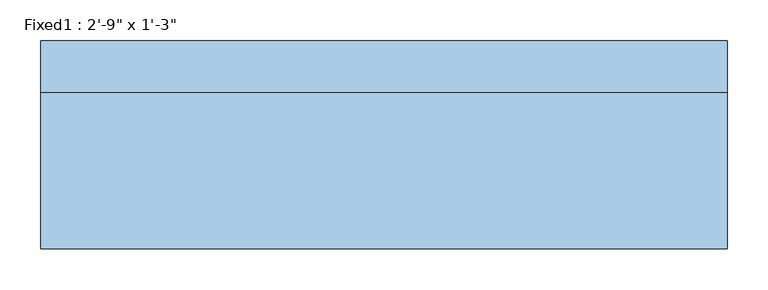
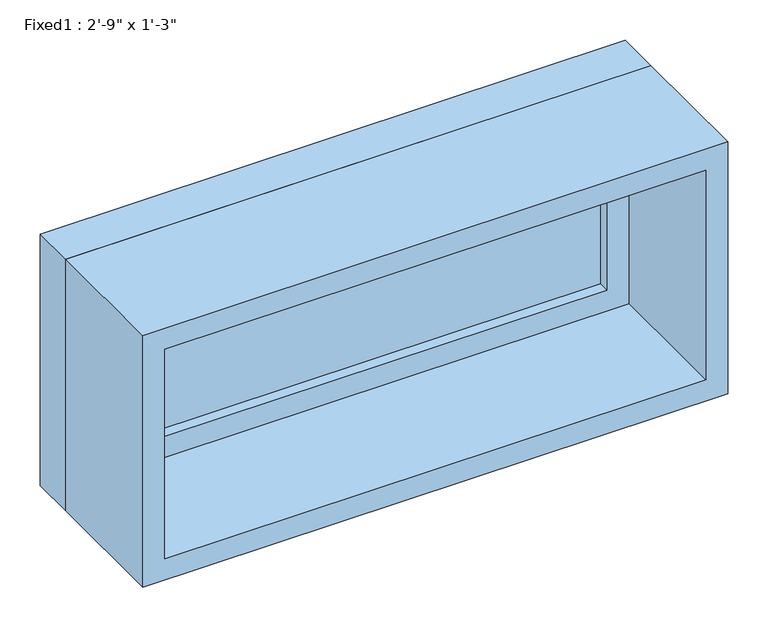
"""IFC4 building model written with IfcOpenShell, lengths in millimetres: window geometry."""

import ifcopenshell
import ifcopenshell.guid

model = None  # the IFC model being written
_history = None  # IfcOwnerHistory: only IFC2X3 demands one
_inside = {}  # id of a spatial element -> (the spatial element, [elements in it])
_under = {}  # id of a project, library or spatial element -> (it, [spatial elements below it])
_declared = {}  # id of a project -> (the project, [libraries it declares])
_typed = {}  # id of a type object -> (the type object, [elements of that type])
_made_of = {}  # id of a material, layer set ... -> (it, [elements and type objects made of it])


def new_model(schema):
    """Start an empty IFC model of exactly this schema.

    Asked for "IFC4X3", IfcOpenShell would pick the latest addendum, in which some entities
    have other attributes; the version numbers below select the first issue.
    IFC2X3 requires an IfcOwnerHistory on every rooted entity: one is made here for all.
    """
    global model, _history
    if schema == "IFC4X3":
        model = ifcopenshell.file(schema_version=(4, 3, 0, 0))
    else:
        model = ifcopenshell.file(schema=schema)
    _inside.clear()
    _under.clear()
    _declared.clear()
    _typed.clear()
    _made_of.clear()
    _history = None
    if model.schema == "IFC2X3":
        org = make("IfcOrganization", Name="unknown")
        user = make(
            "IfcPersonAndOrganization",
            ThePerson=make("IfcPerson", FamilyName="unknown"),
            TheOrganization=org,
        )
        app = make(
            "IfcApplication",
            ApplicationDeveloper=org,
            Version="unknown",
            ApplicationFullName="unknown",
            ApplicationIdentifier="unknown",
        )
        _history = make(
            "IfcOwnerHistory",
            OwningUser=user,
            OwningApplication=app,
            ChangeAction="ADDED",
            CreationDate=0,
        )
    return model


def make(cls, **values):
    """One entity of the class cls with the attributes given. An attribute that is None is left unset."""
    return model.create_entity(
        cls, **{name: value for name, value in values.items() if value is not None}
    )


def rooted(cls, **values):
    """An entity with a GlobalId (a new one), such as an element, a storey or a relation."""
    return make(cls, GlobalId=ifcopenshell.guid.new(), OwnerHistory=_history, **values)


def si_unit(unit_type, name, prefix=None):
    """IfcSIUnit, for example si_unit("LENGTHUNIT", "METRE", prefix="MILLI")."""
    return make("IfcSIUnit", UnitType=unit_type, Prefix=prefix, Name=name)


def assignment(units):
    """IfcUnitAssignment: the units of a project."""
    return None if units is None else make("IfcUnitAssignment", Units=units)


def point(xyz):
    """IfcCartesianPoint."""
    return None if xyz is None else make("IfcCartesianPoint", Coordinates=xyz)


def direction(xyz):
    """IfcDirection."""
    return None if xyz is None else make("IfcDirection", DirectionRatios=xyz)


def frame(location, z_axis=None, x_axis=None):
    """IfcAxis2Placement3D, a coordinate frame: its origin and axes. An axis left out is left unset."""
    return make(
        "IfcAxis2Placement3D",
        Location=point(location),
        Axis=direction(z_axis),
        RefDirection=direction(x_axis),
    )


def origin():
    """The frame at (0, 0, 0) with its axes left unset."""
    return frame((0.0, 0.0, 0.0))


def place(relative_to, where):
    """IfcLocalPlacement: puts the frame where relative to a parent placement (None: the world)."""
    return make(
        "IfcLocalPlacement", PlacementRelTo=relative_to, RelativePlacement=where
    )


def context(
    kind, dimensions, precision=None, world=None, true_north=None, identifier=None
):
    """IfcGeometricRepresentationContext, for example the 3D "Model" context."""
    return make(
        "IfcGeometricRepresentationContext",
        ContextIdentifier=identifier,
        ContextType=kind,
        CoordinateSpaceDimension=dimensions,
        Precision=precision,
        WorldCoordinateSystem=world,
        TrueNorth=true_north,
    )


def project(units=None, contexts=None):
    """IfcProject with its units and contexts."""
    return rooted(
        "IfcProject",
        Name="project",
        RepresentationContexts=contexts,
        UnitsInContext=assignment(units),
    )


def spatial(cls, under=None, at=None, **own):
    """A site, building, storey or space (cls), placed at a placement, below another one or the project."""
    s = rooted(cls, ObjectPlacement=at, **own)
    if under is not None:
        _under.setdefault(under.id(), (under, []))[1].append(s)
    return s


def polyline(points):
    """IfcPolyline through the points."""
    return make("IfcPolyline", Points=[point(p) for p in points])


def outline(outer, holes=None, kind="AREA"):
    """IfcArbitraryClosedProfileDef: a profile drawn as a closed curve; with holes, ...WithVoids."""
    if holes is None:
        return make("IfcArbitraryClosedProfileDef", ProfileType=kind, OuterCurve=outer)
    return make(
        "IfcArbitraryProfileDefWithVoids",
        ProfileType=kind,
        OuterCurve=outer,
        InnerCurves=holes,
    )


def extrude(swept, where, along, depth):
    """IfcExtrudedAreaSolid: the profile swept, set in the frame where, extruded along a direction by depth."""
    return make(
        "IfcExtrudedAreaSolid",
        SweptArea=swept,
        Position=where,
        ExtrudedDirection=direction(along),
        Depth=depth,
    )


def shape(context_of_items, identifier, shape_type, items):
    """IfcShapeRepresentation: the items that make up one representation, for example the "Body"."""
    return make(
        "IfcShapeRepresentation",
        ContextOfItems=context_of_items,
        RepresentationIdentifier=identifier,
        RepresentationType=shape_type,
        Items=items,
    )


def source(mapping_origin, context_of_items, identifier, shape_type, items):
    """IfcRepresentationMap: a shape defined once, which mapped items show again and again."""
    return make(
        "IfcRepresentationMap",
        MappingOrigin=mapping_origin,
        MappedRepresentation=shape(context_of_items, identifier, shape_type, items),
    )


def transform(
    local_origin,
    x_axis=None,
    y_axis=None,
    z_axis=None,
    scale=None,
    scale2=None,
    scale3=None,
    uniform=True,
):
    """IfcCartesianTransformationOperator3D, or its non-uniform kind. x_axis, y_axis, z_axis: its Axis1, 2, 3."""
    if uniform:
        return make(
            "IfcCartesianTransformationOperator3D",
            Axis1=direction(x_axis),
            Axis2=direction(y_axis),
            LocalOrigin=point(local_origin),
            Scale=scale,
            Axis3=direction(z_axis),
        )
    return make(
        "IfcCartesianTransformationOperator3DnonUniform",
        Axis1=direction(x_axis),
        Axis2=direction(y_axis),
        LocalOrigin=point(local_origin),
        Scale=scale,
        Axis3=direction(z_axis),
        Scale2=scale2,
        Scale3=scale3,
    )


def mapped(mapping_source, mapping_target):
    """IfcMappedItem: shows the shape of a source again, moved by a transform."""
    return make(
        "IfcMappedItem", MappingSource=mapping_source, MappingTarget=mapping_target
    )


def made_of(thing, what):
    """Note that an element or type object is made of a material, layer set ...; save() writes the relation."""
    if what is not None:
        _made_of.setdefault(what.id(), (what, []))[1].append(thing)
    return thing


def element(
    cls,
    number,
    at=None,
    inside=None,
    cuts=None,
    type_object=None,
    material=None,
    context=None,
    identifier="Body",
    shape_type=None,
    held_by="IfcProductDefinitionShape",
    body=None,
    shapes=None,
    **own,
):
    """One element of the class cls, such as IfcWall. Its Tag is "e" and its number.

    at: its placement. inside: the storey or other place that contains it. cuts: it is an
    opening in that element (IfcRelVoidsElement). A single representation is given by context,
    identifier, shape_type and body (its items); several are given by shapes. held_by: the class
    of the entity that holds the representations. save() writes the other relations.
    """
    e = rooted(cls, Tag="e%d" % number, ObjectPlacement=at, **own)
    if body is not None:
        shapes = [shape(context, identifier, shape_type, body)]
    if shapes is not None:
        e.Representation = make(held_by, Representations=shapes)
    if inside is not None:
        _inside.setdefault(inside.id(), (inside, []))[1].append(e)
    if cuts is not None:
        rooted(
            "IfcRelVoidsElement", RelatingBuildingElement=cuts, RelatedOpeningElement=e
        )
    if type_object is not None:
        _typed.setdefault(type_object.id(), (type_object, []))[1].append(e)
    return made_of(e, material)


def aggregate(whole, parts):
    """IfcRelAggregates: a whole, such as a stair, and the parts it consists of."""
    return rooted("IfcRelAggregates", RelatingObject=whole, RelatedObjects=parts)


def save(model, path):
    """Write the relations noted so far, then the file.

    IfcRelAggregates (storeys below a building ...), IfcRelContainedInSpatialStructure (elements
    in a storey), IfcRelDefinesByType, IfcRelAssociatesMaterial and IfcRelDeclares: one each for
    every whole, place, type object, material and project.
    """
    for whole, parts in _under.values():
        aggregate(whole, parts)
    for where, things in _inside.values():
        rooted(
            "IfcRelContainedInSpatialStructure",
            RelatedElements=things,
            RelatingStructure=where,
        )
    for kind, things in _typed.values():
        rooted("IfcRelDefinesByType", RelatedObjects=things, RelatingType=kind)
    for what, things in _made_of.values():
        rooted("IfcRelAssociatesMaterial", RelatedObjects=things, RelatingMaterial=what)
    for by, libraries in _declared.values():
        rooted("IfcRelDeclares", RelatingContext=by, RelatedDefinitions=libraries)
    model.write(path)


def window_bf5cd34b(model_context):
    return source(origin(), model_context, "Body", "SweptSolid", [
        extrude(outline(polyline([(317.5, 79.375), (-393.7, 79.375), (-393.7, 92.075), (317.5, 92.075), (317.5, 79.375)])), frame((0.0, 0.0, 977.9), z_axis=(0.0, 0.0, 1.0), x_axis=(1.0, 0.0, 0.0)), (0.0, 0.0, 1.0), 254.0),
        extrude(outline(polyline([(1276.35, -438.15), (933.45, -438.15), (933.45, 361.95), (1276.35, 361.95), (1276.35, -438.15)]), holes=[polyline([(1231.9, -393.7), (1231.9, 317.5), (977.9, 317.5), (977.9, -393.7), (1231.9, -393.7)])]), frame((0.0, 63.5, 0.0), z_axis=(0.0, 1.0, 0.0), x_axis=(0.0, 0.0, 1.0)), (0.0, 0.0, 1.0), 44.45),
        extrude(outline(polyline([(1295.4, -457.2), (914.4, -457.2), (914.4, 381.0), (1295.4, 381.0), (1295.4, -457.2)]), holes=[polyline([(1263.65, -425.45), (1263.65, 349.25), (946.15, 349.25), (946.15, -425.45), (1263.65, -425.45)])]), frame((0.0, -127.0, 0.0), z_axis=(0.0, 1.0, 0.0), x_axis=(0.0, 0.0, 1.0)), (0.0, 0.0, 1.0), 190.5),
        extrude(outline(polyline([(1295.4, 381.0), (1295.4, -457.2), (914.4, -457.2), (914.4, 381.0), (1295.4, 381.0)]), holes=[polyline([(1276.35, 361.95), (933.45, 361.95), (933.45, -438.15), (1276.35, -438.15), (1276.35, 361.95)])]), frame((0.0, 63.5, 0.0), z_axis=(0.0, 1.0, 0.0), x_axis=(0.0, 0.0, 1.0)), (0.0, 0.0, 1.0), 63.5),
    ])


if __name__ == "__main__":
    model = new_model("IFC4")
    model_context = context("Model", 3, world=origin())
    ifc_project = project(units=[si_unit("LENGTHUNIT", "METRE", prefix="MILLI")], contexts=[model_context])
    site = spatial("IfcSite", under=ifc_project)
    building = spatial("IfcBuilding", under=site)
    placement = place(None, origin())
    window_shape = window_bf5cd34b(model_context)
    element("IfcWindow", 1, ObjectType="Fixed1 : 2'-9\" x 1'-3\"", at=placement, inside=building, context=model_context, shape_type="MappedRepresentation", body=[
        mapped(window_shape, transform((0.0, 0.0, 0.0), x_axis=(1.0, 0.0, 0.0), y_axis=(0.0, 1.0, 0.0), z_axis=(0.0, 0.0, 1.0))),
    ])
    save(model, "model.ifc")

# Revit data of these elements
# Type "Fixed1 : 2'-9\" x 1'-3\""
#   Type Mark = "29"
#   Construction Type Id = "GSP4R"
#   Assembly Code = "B2020100"
#   Analytic Construction = "1/8 in Pilkington single glazing"
#   Visual Light Transmittance = 0.9
#   Solar Heat Gain Coefficient = 0.78
#   Heat Transfer Coefficient (U) = 3.6886 W/(m²·K)
#   Height = 1' - 3"
#   Default Sill Height = 3' - 0"
#   Width = 2' - 9"
#   Window Inset = 0' - 0 3/4"
#   Glass Pane Material = Glass
#   Sash Material = Sash
#   Wall Closure = (empty or 0)
# Element 1 (IfcWindow, "Fixed1 : 2'-9\" x 1'-3\"")
#   Materials on its faces: "Sash", "Glass"
# Materials
#   "Glass": class "Glass", colour RGB 218 227 224, transparency 0.85, Description = "Soda Lime Glass", Cost = 0
#   "Sash": class "Wood", colour RGB 224 178 126, transparency 0, Cost = 0
